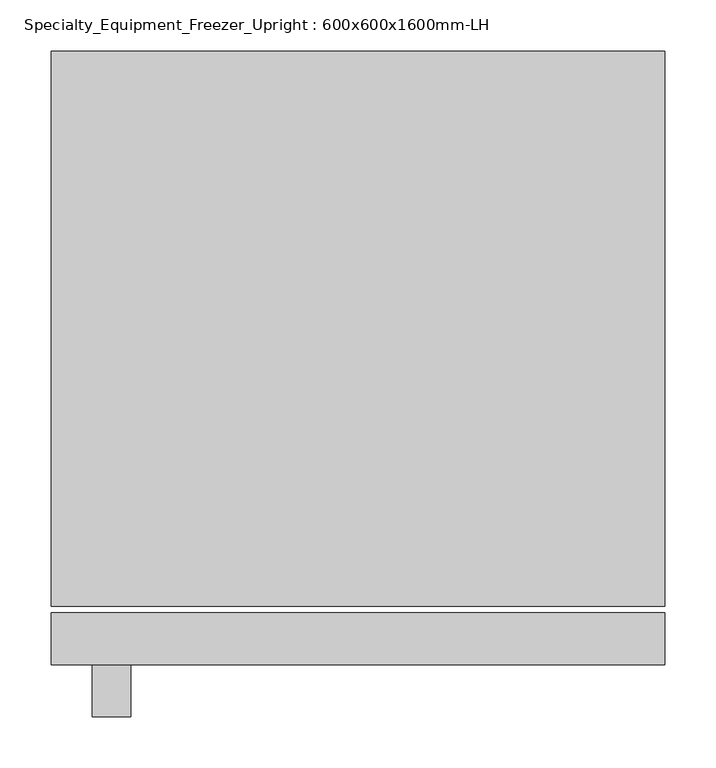
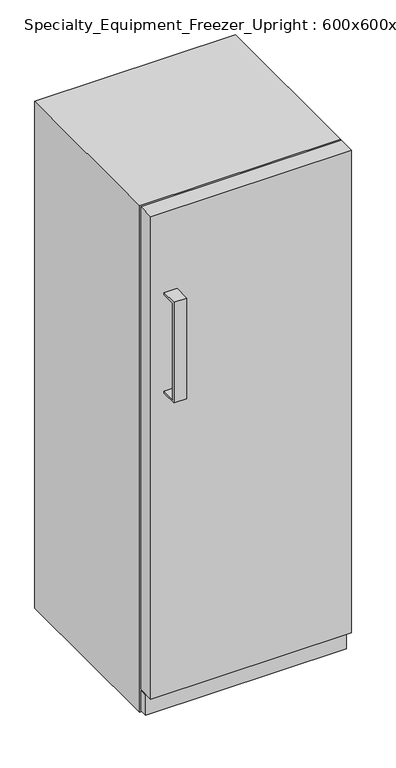
"""IFC4 building model written with IfcOpenShell, lengths in millimetres: proxy geometry, Specialty_Equipment_Freezer_Upright : 600x600x1600mm-LH."""

import ifcopenshell
import ifcopenshell.guid

model = None  # the IFC model being written
_history = None  # IfcOwnerHistory: only IFC2X3 demands one
_inside = {}  # id of a spatial element -> (the spatial element, [elements in it])
_under = {}  # id of a project, library or spatial element -> (it, [spatial elements below it])
_declared = {}  # id of a project -> (the project, [libraries it declares])
_typed = {}  # id of a type object -> (the type object, [elements of that type])
_made_of = {}  # id of a material, layer set ... -> (it, [elements and type objects made of it])


def new_model(schema):
    """Start an empty IFC model of exactly this schema.

    Asked for "IFC4X3", IfcOpenShell would pick the latest addendum, in which some entities
    have other attributes; the version numbers below select the first issue.
    IFC2X3 requires an IfcOwnerHistory on every rooted entity: one is made here for all.
    """
    global model, _history
    if schema == "IFC4X3":
        model = ifcopenshell.file(schema_version=(4, 3, 0, 0))
    else:
        model = ifcopenshell.file(schema=schema)
    _inside.clear()
    _under.clear()
    _declared.clear()
    _typed.clear()
    _made_of.clear()
    _history = None
    if model.schema == "IFC2X3":
        org = make("IfcOrganization", Name="unknown")
        user = make(
            "IfcPersonAndOrganization",
            ThePerson=make("IfcPerson", FamilyName="unknown"),
            TheOrganization=org,
        )
        app = make(
            "IfcApplication",
            ApplicationDeveloper=org,
            Version="unknown",
            ApplicationFullName="unknown",
            ApplicationIdentifier="unknown",
        )
        _history = make(
            "IfcOwnerHistory",
            OwningUser=user,
            OwningApplication=app,
            ChangeAction="ADDED",
            CreationDate=0,
        )
    return model


def make(cls, **values):
    """One entity of the class cls with the attributes given. An attribute that is None is left unset."""
    return model.create_entity(
        cls, **{name: value for name, value in values.items() if value is not None}
    )


def rooted(cls, **values):
    """An entity with a GlobalId (a new one), such as an element, a storey or a relation."""
    return make(cls, GlobalId=ifcopenshell.guid.new(), OwnerHistory=_history, **values)


def si_unit(unit_type, name, prefix=None):
    """IfcSIUnit, for example si_unit("LENGTHUNIT", "METRE", prefix="MILLI")."""
    return make("IfcSIUnit", UnitType=unit_type, Prefix=prefix, Name=name)


def assignment(units):
    """IfcUnitAssignment: the units of a project."""
    return None if units is None else make("IfcUnitAssignment", Units=units)


def point(xyz):
    """IfcCartesianPoint."""
    return None if xyz is None else make("IfcCartesianPoint", Coordinates=xyz)


def direction(xyz):
    """IfcDirection."""
    return None if xyz is None else make("IfcDirection", DirectionRatios=xyz)


def frame(location, z_axis=None, x_axis=None):
    """IfcAxis2Placement3D, a coordinate frame: its origin and axes. An axis left out is left unset."""
    return make(
        "IfcAxis2Placement3D",
        Location=point(location),
        Axis=direction(z_axis),
        RefDirection=direction(x_axis),
    )


def origin():
    """The frame at (0, 0, 0) with its axes left unset."""
    return frame((0.0, 0.0, 0.0))


def origin_with_axes():
    """The frame at (0, 0, 0) with the z axis (0, 0, 1) and the x axis (1, 0, 0) written out."""
    return frame((0.0, 0.0, 0.0), z_axis=(0.0, 0.0, 1.0), x_axis=(1.0, 0.0, 0.0))


def place(relative_to, where):
    """IfcLocalPlacement: puts the frame where relative to a parent placement (None: the world)."""
    return make(
        "IfcLocalPlacement", PlacementRelTo=relative_to, RelativePlacement=where
    )


def context(
    kind, dimensions, precision=None, world=None, true_north=None, identifier=None
):
    """IfcGeometricRepresentationContext, for example the 3D "Model" context."""
    return make(
        "IfcGeometricRepresentationContext",
        ContextIdentifier=identifier,
        ContextType=kind,
        CoordinateSpaceDimension=dimensions,
        Precision=precision,
        WorldCoordinateSystem=world,
        TrueNorth=true_north,
    )


def project(units=None, contexts=None):
    """IfcProject with its units and contexts."""
    return rooted(
        "IfcProject",
        Name="project",
        RepresentationContexts=contexts,
        UnitsInContext=assignment(units),
    )


def spatial(cls, under=None, at=None, **own):
    """A site, building, storey or space (cls), placed at a placement, below another one or the project."""
    s = rooted(cls, ObjectPlacement=at, **own)
    if under is not None:
        _under.setdefault(under.id(), (under, []))[1].append(s)
    return s


def polyline(points):
    """IfcPolyline through the points."""
    return make("IfcPolyline", Points=[point(p) for p in points])


def outline(outer, holes=None, kind="AREA"):
    """IfcArbitraryClosedProfileDef: a profile drawn as a closed curve; with holes, ...WithVoids."""
    if holes is None:
        return make("IfcArbitraryClosedProfileDef", ProfileType=kind, OuterCurve=outer)
    return make(
        "IfcArbitraryProfileDefWithVoids",
        ProfileType=kind,
        OuterCurve=outer,
        InnerCurves=holes,
    )


def extrude(swept, where, along, depth):
    """IfcExtrudedAreaSolid: the profile swept, set in the frame where, extruded along a direction by depth."""
    return make(
        "IfcExtrudedAreaSolid",
        SweptArea=swept,
        Position=where,
        ExtrudedDirection=direction(along),
        Depth=depth,
    )


def shape(context_of_items, identifier, shape_type, items):
    """IfcShapeRepresentation: the items that make up one representation, for example the "Body"."""
    return make(
        "IfcShapeRepresentation",
        ContextOfItems=context_of_items,
        RepresentationIdentifier=identifier,
        RepresentationType=shape_type,
        Items=items,
    )


def source(mapping_origin, context_of_items, identifier, shape_type, items):
    """IfcRepresentationMap: a shape defined once, which mapped items show again and again."""
    return make(
        "IfcRepresentationMap",
        MappingOrigin=mapping_origin,
        MappedRepresentation=shape(context_of_items, identifier, shape_type, items),
    )


def transform(
    local_origin,
    x_axis=None,
    y_axis=None,
    z_axis=None,
    scale=None,
    scale2=None,
    scale3=None,
    uniform=True,
):
    """IfcCartesianTransformationOperator3D, or its non-uniform kind. x_axis, y_axis, z_axis: its Axis1, 2, 3."""
    if uniform:
        return make(
            "IfcCartesianTransformationOperator3D",
            Axis1=direction(x_axis),
            Axis2=direction(y_axis),
            LocalOrigin=point(local_origin),
            Scale=scale,
            Axis3=direction(z_axis),
        )
    return make(
        "IfcCartesianTransformationOperator3DnonUniform",
        Axis1=direction(x_axis),
        Axis2=direction(y_axis),
        LocalOrigin=point(local_origin),
        Scale=scale,
        Axis3=direction(z_axis),
        Scale2=scale2,
        Scale3=scale3,
    )


def mapped(mapping_source, mapping_target):
    """IfcMappedItem: shows the shape of a source again, moved by a transform."""
    return make(
        "IfcMappedItem", MappingSource=mapping_source, MappingTarget=mapping_target
    )


def made_of(thing, what):
    """Note that an element or type object is made of a material, layer set ...; save() writes the relation."""
    if what is not None:
        _made_of.setdefault(what.id(), (what, []))[1].append(thing)
    return thing


def element(
    cls,
    number,
    at=None,
    inside=None,
    cuts=None,
    type_object=None,
    material=None,
    context=None,
    identifier="Body",
    shape_type=None,
    held_by="IfcProductDefinitionShape",
    body=None,
    shapes=None,
    **own,
):
    """One element of the class cls, such as IfcWall. Its Tag is "e" and its number.

    at: its placement. inside: the storey or other place that contains it. cuts: it is an
    opening in that element (IfcRelVoidsElement). A single representation is given by context,
    identifier, shape_type and body (its items); several are given by shapes. held_by: the class
    of the entity that holds the representations. save() writes the other relations.
    """
    e = rooted(cls, Tag="e%d" % number, ObjectPlacement=at, **own)
    if body is not None:
        shapes = [shape(context, identifier, shape_type, body)]
    if shapes is not None:
        e.Representation = make(held_by, Representations=shapes)
    if inside is not None:
        _inside.setdefault(inside.id(), (inside, []))[1].append(e)
    if cuts is not None:
        rooted(
            "IfcRelVoidsElement", RelatingBuildingElement=cuts, RelatedOpeningElement=e
        )
    if type_object is not None:
        _typed.setdefault(type_object.id(), (type_object, []))[1].append(e)
    return made_of(e, material)


def aggregate(whole, parts):
    """IfcRelAggregates: a whole, such as a stair, and the parts it consists of."""
    return rooted("IfcRelAggregates", RelatingObject=whole, RelatedObjects=parts)


def save(model, path):
    """Write the relations noted so far, then the file.

    IfcRelAggregates (storeys below a building ...), IfcRelContainedInSpatialStructure (elements
    in a storey), IfcRelDefinesByType, IfcRelAssociatesMaterial and IfcRelDeclares: one each for
    every whole, place, type object, material and project.
    """
    for whole, parts in _under.values():
        aggregate(whole, parts)
    for where, things in _inside.values():
        rooted(
            "IfcRelContainedInSpatialStructure",
            RelatedElements=things,
            RelatingStructure=where,
        )
    for kind, things in _typed.values():
        rooted("IfcRelDefinesByType", RelatedObjects=things, RelatingType=kind)
    for what, things in _made_of.values():
        rooted("IfcRelAssociatesMaterial", RelatedObjects=things, RelatingMaterial=what)
    for by, libraries in _declared.values():
        rooted("IfcRelDeclares", RelatingContext=by, RelatedDefinitions=libraries)
    model.write(path)


def specialty_equipment_freezer_upright_600x600x1600mm_lh_8c2ecadc(model_context):
    return source(origin(), model_context, "Body", "SweptSolid", [
        extrude(outline(polyline([(-314.6760285, 1339.65), (-359.1260285, 1339.65), (-359.1260285, 1034.85), (-314.6760285, 1034.85), (-314.6760285, 1028.5154683), (-365.4760285, 1028.5154683), (-365.4760285, 1346.0), (-314.6760285, 1346.0), (-314.6760285, 1339.65)])), frame((-260.0, 0.0, 0.0), z_axis=(1.0, 0.0, 0.0), x_axis=(0.0, 1.0, 0.0)), (0.0, 0.0, 1.0), 38.1),
        extrude(outline(polyline([(300.0, -263.8760285), (300.0, -289.2760285), (-300.0, -289.2760285), (-300.0, -263.8760285), (300.0, -263.8760285)])), frame((0.0, 0.0, 9.3816357), z_axis=(0.0, 0.0, 1.0), x_axis=(1.0, 0.0, 0.0)), (0.0, 0.0, 1.0), 63.5),
        extrude(outline(polyline([(300.0, -263.8760285), (300.0, -314.6760285), (-300.0, -314.6760285), (-300.0, -263.8760285), (300.0, -263.8760285)])), frame((0.0, 0.0, 76.2), z_axis=(0.0, 0.0, 1.0), x_axis=(1.0, 0.0, 0.0)), (0.0, 0.0, 1.0), 1523.8),
        extrude(outline(polyline([(300.0, 285.3239715), (300.0, -257.5260285), (-300.0, -257.5260285), (-300.0, 285.3239715), (300.0, 285.3239715)])), origin_with_axes(), (0.0, 0.0, 1.0), 1600.0),
    ])


if __name__ == "__main__":
    model = new_model("IFC4")
    model_context = context("Model", 3, world=origin())
    ifc_project = project(units=[si_unit("LENGTHUNIT", "METRE", prefix="MILLI")], contexts=[model_context])
    site = spatial("IfcSite", under=ifc_project)
    building = spatial("IfcBuilding", under=site)
    placement = place(None, origin())
    specialty_equipment_freezer_upright_600x600x1600mm_lh_shape = specialty_equipment_freezer_upright_600x600x1600mm_lh_8c2ecadc(model_context)
    element("IfcBuildingElementProxy", 1, Name="Specialty_Equipment_Freezer_Upright : 600x600x1600mm-LH", ObjectType="Specialty_Equipment_Freezer_Upright : 600x600x1600mm-LH", at=placement, inside=building, context=model_context, shape_type="MappedRepresentation", body=[
        mapped(specialty_equipment_freezer_upright_600x600x1600mm_lh_shape, transform((0.0, 0.0, 0.0), x_axis=(1.0, 0.0, 0.0), y_axis=(0.0, 1.0, 0.0), z_axis=(0.0, 0.0, 1.0))),
    ])
    save(model, "model.ifc")

# Revit data of these elements
# Type "Specialty_Equipment_Freezer_Upright : 600x600x1600mm-LH"
#   Type IfcGUID = "1aRjrFHzDDvwx1NU_3WgZx"
#   Classification.Uniclass.EF.Number = "EF_40_40"
#   Classification.Uniclass.EF.Description = "Equipment"
#   Keynote = "N10"
#   Assembly Code = "E1090400"
#   Depth = 0.6 m
#   Handle = 0.04 m
#   Height = 1.6 m
#   Rear Clearance = 0.05 m
#   Width = 0.6 m
#   Material = Metal - Paint Finish - Ivory, Glossy
#   Default Elevation = 0
# Element 1 (IfcBuildingElementProxy, "Specialty_Equipment_Freezer_Upright : 600x600x1600mm-LH")
#   Materials on its faces: "Metal - Paint Finish - Ivory, Glossy", "Metal - Chrome", "Metal - Paint Finish - Black, Glossy"
# Materials
#   "Metal - Paint Finish - Ivory, Glossy": class "Paint", colour RGB 247 247 239, transparency 0
#   "Metal - Chrome": class "Metal", colour RGB 247 247 247, transparency 0
#   "Metal - Paint Finish - Black, Glossy": class "Metal", colour RGB 0 0 0, transparency 0
